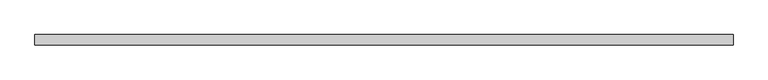
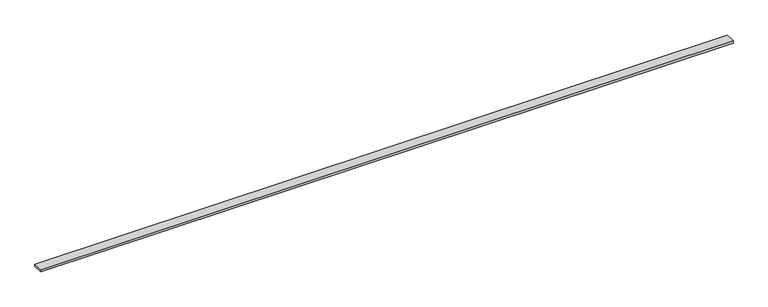
"""IFC4 building model written with IfcOpenShell, lengths in millimetres: proxy geometry, Generic Models 7:Generic Models 1:337419:Generic Models 1:337419 : Generic Models 7:Generic Models 1:337419:34 : Generic Models 7:Generic Models 1:337419:Generic Models 1:337419 : Generic Models 7:Generic Models 1:337419:301336."""

from ifc_helpers import new_model, si_unit, frame, origin, place, context, project, spatial, polyline, outline, extrude, source, transform, mapped, element, save


def generic_models_3fad15a1(model_context):
    return source(origin(), model_context, "Body", "SweptSolid", [
        extrude(outline(polyline([(-578981.6413841, 6129.1390625), (-578981.6413841, 6175.1765625), (-578797.4913841, 6165.5256699), (-578797.4913841, 6129.1390625), (-578981.6413841, 6129.1390625)])), frame((560419.6367239, 0.0, 0.0), z_axis=(1.0, 0.0, 0.0), x_axis=(0.0, 1.0, 0.0)), (0.0, 0.0, 1.0), 12477.75),
    ])


if __name__ == "__main__":
    model = new_model("IFC4")
    model_context = context("Model", 3, world=origin())
    ifc_project = project(units=[si_unit("LENGTHUNIT", "METRE", prefix="MILLI")], contexts=[model_context])
    site = spatial("IfcSite", under=ifc_project)
    building = spatial("IfcBuilding", under=site)
    placement = place(None, origin())
    generic_models_shape = generic_models_3fad15a1(model_context)
    element("IfcBuildingElementProxy", 1, Name="Generic Models 7:Generic Models 1:337419:Generic Models 1:337419 : Generic Models 7:Generic Models 1:337419:34 : Generic Models 7:Generic Models 1:337419:Generic Models 1:337419 : Generic Models 7:Generic Models 1:337419:301336", ObjectType="Generic Models 7:Generic Models 1:337419:Generic Models 1:337419 : Generic Models 7:Generic Models 1:337419:34 : Generic Models 7:Generic Models 1:337419:Generic Models 1:337419 : Generic Models 7:Generic Models 1:337419:301336", at=placement, inside=building, context=model_context, shape_type="MappedRepresentation", body=[
        mapped(generic_models_shape, transform((0.0, 0.0, 0.0), x_axis=(1.0, 0.0, 0.0), y_axis=(0.0, 1.0, 0.0), z_axis=(0.0, 0.0, 1.0))),
    ])
    save(model, "model.ifc")

# Revit data of these elements
# Type "Generic Models 7:Generic Models 1:337419:Generic Models 1:337419 : Generic Models 7:Generic Models 1:337419:34 : Generic Models 7:Generic Models 1:337419:Generic Models 1:337419 : Generic Models 7:Generic Models 1:337419:301336"
#   NameOverride = "Generic Models 7:Generic Models 1:337419:Generic Models 1:337419 : Generic Models 7:Generic Models 1:337419:301336"
#   ObjectTypeOverride = "Generic Models 1:337419 : Generic Models 7:Generic Models 1:337419"
#   Reference = "Generic Models 1"
#   Tag = "301336"
# Element 1 (IfcBuildingElementProxy, "Generic Models 7:Generic Models 1:337419:Generic Models 1:337419 : Generic Models 7:Generic Models 1:337419:34 : Generic Models 7:Generic Models 1:337419:Generic Models 1:337419 : Generic Models 7:Generic Models 1:337419:301336")
#   Materials on its faces: "BLOCKING - SIZE AS NEC."
# Materials
#   "BLOCKING - SIZE AS NEC.": class "Wood", colour RGB 144 113 62, transparency 0, Description = "Pinus Echinata", Cost = 0
